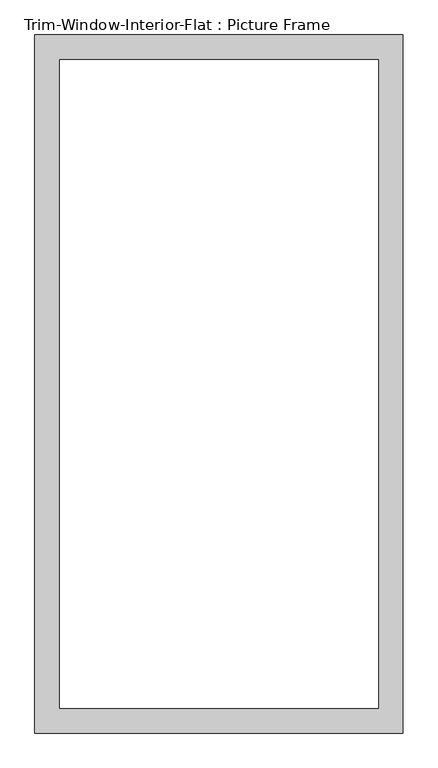
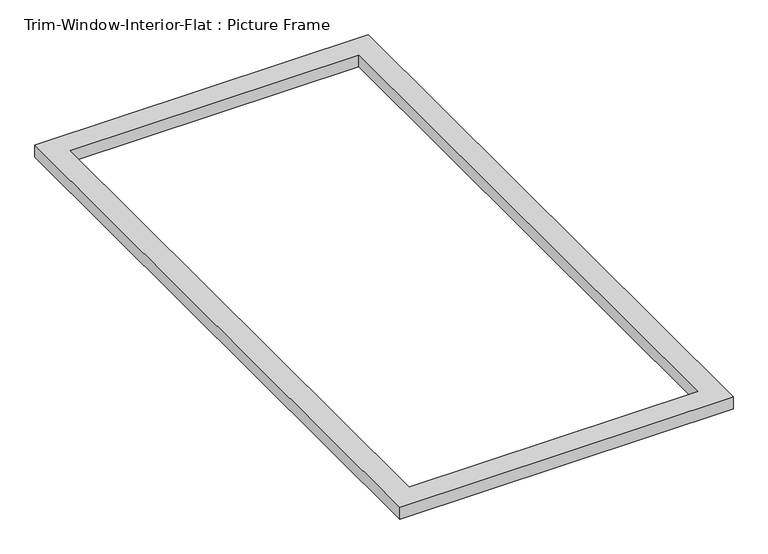
"""IFC4 building model written with IfcOpenShell, lengths in millimetres: proxy geometry, Trim-Window-Interior-Flat : Picture Frame."""

from ifc_helpers import new_model, si_unit, origin, origin_with_axes, place, context, project, spatial, polyline, outline, extrude, source, transform, mapped, element, save


def trim_window_interior_flat_picture_frame_aab62eac(model_context):
    return source(origin(), model_context, "Body", "SweptSolid", [
        extrude(outline(polyline([(425.45, -44.45), (-425.45, -44.45), (-425.45, 1568.45), (425.45, 1568.45), (425.45, -44.45)]), holes=[polyline([(368.3, 12.7), (368.3, 1511.3), (-368.3, 1511.3), (-368.3, 12.7), (368.3, 12.7)])]), origin_with_axes(), (0.0, 0.0, 1.0), 31.75),
    ])


if __name__ == "__main__":
    model = new_model("IFC4")
    model_context = context("Model", 3, world=origin())
    ifc_project = project(units=[si_unit("LENGTHUNIT", "METRE", prefix="MILLI")], contexts=[model_context])
    site = spatial("IfcSite", under=ifc_project)
    building = spatial("IfcBuilding", under=site)
    placement = place(None, origin())
    trim_window_interior_flat_picture_frame_shape = trim_window_interior_flat_picture_frame_aab62eac(model_context)
    element("IfcBuildingElementProxy", 1, Name="Trim-Window-Interior-Flat : Picture Frame", ObjectType="Trim-Window-Interior-Flat : Picture Frame", at=placement, inside=building, context=model_context, shape_type="MappedRepresentation", body=[
        mapped(trim_window_interior_flat_picture_frame_shape, transform((0.0, 0.0, 0.0), x_axis=(1.0, 0.0, 0.0), y_axis=(0.0, 1.0, 0.0), z_axis=(0.0, 0.0, 1.0))),
    ])
    save(model, "model.ifc")

# Revit data of these elements
# Type "Trim-Window-Interior-Flat : Picture Frame"
#   Trim Thickness_Picture Frame = 0' - 1 1/4"
#   Trim Width = 0' - 2 1/4"
#   Trim Thickness_with Sill = 0' - 0 3/4"
#   Sill Thickness = 0' - 1 1/4"
#   Opening Width [instance default] = 2' - 0"
#   Opening Height [instance default] = 3' - 0"
#   Default Elevation = 4' - 0"
#   Sill = no
#   Picture Frame = yes
#   Trim Material [instance default] = none
# Element 1 (IfcBuildingElementProxy, "Trim-Window-Interior-Flat : Picture Frame")
#   Opening Width = 2' - 6"
#   Opening Height = 5' - 0"
#   Trim Material = Wood - Stained
#   Materials on its faces: "Wood - Stained"
# Materials
#   "Wood - Stained": class "Wood", colour RGB 224 178 126, transparency 0, Cost = 0
